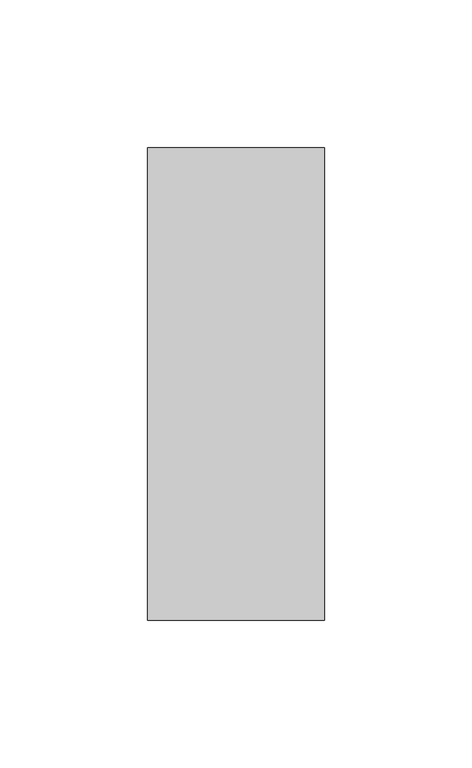
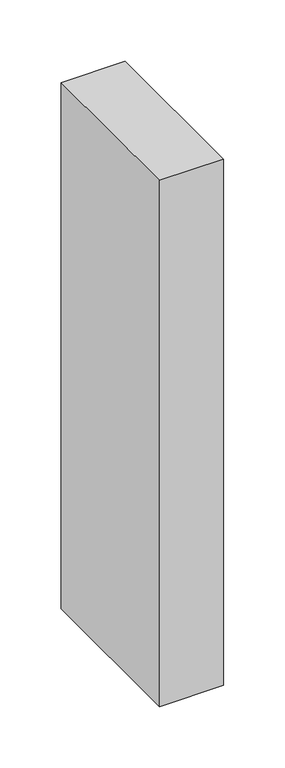
"""IFC4 building model written with IfcOpenShell, lengths in millimetres: column geometry, Madeira de lei-Coluna : Pontalete 6X16cm."""

from ifc_helpers import new_model, si_unit, frame, origin, place, context, project, spatial, polyline, outline, extrude, source, transform, mapped, element, save


def column_f3930958(model_context):
    return source(origin(), model_context, "Body", "SweptSolid", [
        extrude(outline(polyline([(30.0, 80.0), (30.0, -80.0), (-30.0, -80.0), (-30.0, 80.0), (30.0, 80.0)])), frame((0.0, 0.0, 4460.0), z_axis=(0.0, 0.0, 1.0), x_axis=(1.0, 0.0, 0.0)), (0.0, 0.0, 1.0), 522.9),
    ])


if __name__ == "__main__":
    model = new_model("IFC4")
    model_context = context("Model", 3, world=origin())
    ifc_project = project(units=[si_unit("LENGTHUNIT", "METRE", prefix="MILLI")], contexts=[model_context])
    site = spatial("IfcSite", under=ifc_project)
    building = spatial("IfcBuilding", under=site)
    placement = place(None, origin())
    column_shape = column_f3930958(model_context)
    element("IfcColumn", 1, ObjectType="Madeira de lei-Coluna : Pontalete 6X16cm", at=placement, inside=building, context=model_context, shape_type="MappedRepresentation", body=[
        mapped(column_shape, transform((0.0, 0.0, 0.0), x_axis=(1.0, 0.0, 0.0), y_axis=(0.0, 1.0, 0.0), z_axis=(0.0, 0.0, 1.0))),
    ])
    save(model, "model.ifc")

# Revit data of these elements
# Type "Madeira de lei-Coluna : Pontalete 6X16cm"
#   A = 0.01952 m²
#   b = 0.06 m
#   d = 0.16 m
#   Structural Material [instance default] = none
#   Assembly Code = ""
# Element 1 (IfcColumn, "Madeira de lei-Coluna : Pontalete 6X16cm")
#   Structural Material = .MADEIRAMENTO
#   Materials on its faces: ".MADEIRAMENTO"
# Materials
#   ".MADEIRAMENTO": class ".CC_MADEIRAS", colour RGB 212 179 113, transparency 0, Cost = 0
